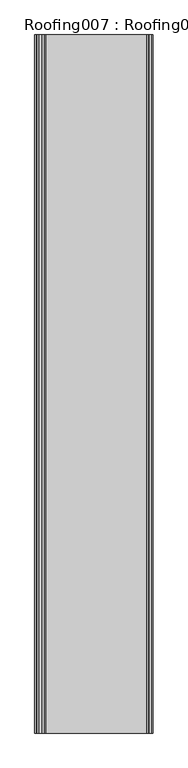
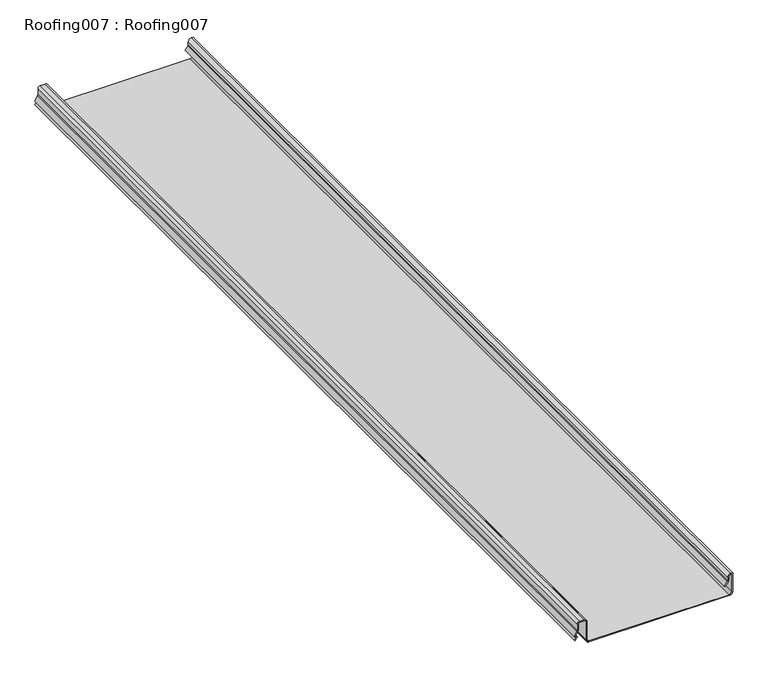
"""IFC4 building model written with IfcOpenShell, lengths in millimetres: proxy geometry, Roofing007 : Roofing007."""

from ifc_helpers import new_model, si_unit, point, frame, frame_2d, origin, place, context, project, spatial, polyline, circle_curve, trimmed, segment, composite_curve, outline, extrude, source, transform, mapped, element, save


def roofing007_roofing007_e383adbc(model_context):
    return source(origin(), model_context, "Body", "SweptSolid", [
        extrude(outline(composite_curve([segment(trimmed(circle_curve(frame_2d((42571.8416239, -858.0818689)), 5.08), [point((42568.8585944, -853.969943))], [point((42571.8416239, -853.0018689))], False, "CARTESIAN"), True, "CONTINUOUS"), segment(polyline([(42571.8416239, -853.0018689), (42578.5981823, -853.0018689)]), True, "CONTINUOUS"), segment(trimmed(circle_curve(frame_2d((42578.5981823, -847.9218689)), 5.08), [point((42578.5981823, -853.0018689))], [point((42583.6781823, -847.9218689))], True, "CARTESIAN"), True, "CONTINUOUS"), segment(polyline([(42583.6781823, -847.9218689), (42583.6781823, -846.3270642), (42543.9409948, -846.3270642)]), True, "CONTINUOUS"), segment(trimmed(circle_curve(frame_2d((42543.9409948, -851.4070642)), 5.08), [point((42543.9409948, -846.3270642))], [point((42538.8609948, -851.4070642))], True, "CARTESIAN"), True, "CONTINUOUS"), segment(polyline([(42538.8609948, -851.4070642), (42538.8609948, -1151.6811463)]), True, "CONTINUOUS"), segment(trimmed(circle_curve(frame_2d((42543.9409948, -1151.6811463)), 5.08), [point((42538.8609948, -1151.6811463))], [point((42543.9409948, -1156.7611463))], True, "CARTESIAN"), True, "CONTINUOUS"), segment(polyline([(42543.9409948, -1156.7611463), (42585.5544323, -1156.7611463)]), True, "CONTINUOUS"), segment(trimmed(circle_curve(frame_2d((42585.5544323, -1161.8411463)), 5.08), [point((42585.5544323, -1156.7611463))], [point((42590.6344323, -1161.8411463))], False, "CARTESIAN"), True, "CONTINUOUS"), segment(polyline([(42590.6344323, -1161.8411463), (42590.6344323, -1171.8489232)]), True, "CONTINUOUS"), segment(trimmed(circle_curve(frame_2d((42585.5544323, -1171.8489232)), 5.08), [point((42590.6344323, -1171.8489232))], [point((42585.5544323, -1176.9289232))], False, "CARTESIAN"), True, "CONTINUOUS"), segment(polyline([(42585.5544323, -1176.9289232), (42572.3718581, -1176.9289232)]), True, "CONTINUOUS"), segment(trimmed(circle_curve(frame_2d((42572.3718581, -1182.0089232)), 5.08), [point((42572.3718581, -1176.9289232))], [point((42569.8678467, -1177.5889315))], True, "CARTESIAN"), True, "CONTINUOUS"), segment(polyline([(42569.8678467, -1177.5889315), (42559.3102135, -1183.5700364), (42556.8688073, -1179.4059739), (42551.2672448, -1183.4049974), (42550.1051711, -1181.7772429), (42557.4874863, -1176.5069185), (42560.0388845, -1180.8585833), (42568.8820154, -1175.8487773)]), True, "CONTINUOUS"), segment(trimmed(circle_curve(frame_2d((42572.3718581, -1182.0089232)), 7.08), [point((42568.8820154, -1175.8487773))], [point((42572.3718581, -1174.9289232))], False, "CARTESIAN"), True, "CONTINUOUS"), segment(polyline([(42572.3718581, -1174.9289232), (42585.5544323, -1174.9289232)]), True, "CONTINUOUS"), segment(trimmed(circle_curve(frame_2d((42585.5544323, -1171.8489232)), 3.08), [point((42585.5544323, -1174.9289232))], [point((42588.6344323, -1171.8489232))], True, "CARTESIAN"), True, "CONTINUOUS"), segment(polyline([(42588.6344323, -1171.8489232), (42588.6344323, -1161.8411463)]), True, "CONTINUOUS"), segment(trimmed(circle_curve(frame_2d((42585.5544323, -1161.8411463)), 3.08), [point((42588.6344323, -1161.8411463))], [point((42585.5544323, -1158.7611463))], True, "CARTESIAN"), True, "CONTINUOUS"), segment(polyline([(42585.5544323, -1158.7611463), (42543.9409948, -1158.7611463)]), True, "CONTINUOUS"), segment(trimmed(circle_curve(frame_2d((42543.9409948, -1151.6811463)), 7.08), [point((42543.9409948, -1158.7611463))], [point((42536.8609948, -1151.6811463))], False, "CARTESIAN"), True, "CONTINUOUS"), segment(polyline([(42536.8609948, -1151.6811463), (42536.8609948, -851.4070642)]), True, "CONTINUOUS"), segment(trimmed(circle_curve(frame_2d((42543.9409948, -851.4070642)), 7.08), [point((42536.8609948, -851.4070642))], [point((42543.9409948, -844.3270642))], False, "CARTESIAN"), True, "CONTINUOUS"), segment(polyline([(42543.9409948, -844.3270642), (42585.6781823, -844.3270642), (42585.6781823, -847.9218689)]), True, "CONTINUOUS"), segment(trimmed(circle_curve(frame_2d((42578.5981823, -847.9218689)), 7.08), [point((42585.6781823, -847.9218689))], [point((42578.5981823, -855.0018689))], False, "CARTESIAN"), True, "CONTINUOUS"), segment(polyline([(42578.5981823, -855.0018689), (42571.8416239, -855.0018689)]), True, "CONTINUOUS"), segment(trimmed(circle_curve(frame_2d((42571.8416239, -858.0818689)), 3.08), [point((42571.8416239, -855.0018689))], [point((42570.0330155, -855.5888115))], True, "CARTESIAN"), True, "CONTINUOUS"), segment(polyline([(42570.0330155, -855.5888115), (42561.5588533, -861.7364601), (42560.3844323, -860.1175916), (42568.8585944, -853.969943)]), True, "CONTINUOUS")], self_intersect=False)), frame((0.0, -1052.8906574, 0.0), z_axis=(0.0, 1.0, 0.0), x_axis=(0.0, 0.0, 1.0)), (0.0, 0.0, 1.0), 2000.0),
    ])


if __name__ == "__main__":
    model = new_model("IFC4")
    model_context = context("Model", 3, world=origin())
    ifc_project = project(units=[si_unit("LENGTHUNIT", "METRE", prefix="MILLI")], contexts=[model_context])
    site = spatial("IfcSite", under=ifc_project)
    building = spatial("IfcBuilding", under=site)
    placement = place(None, origin())
    roofing007_roofing007_shape = roofing007_roofing007_e383adbc(model_context)
    element("IfcBuildingElementProxy", 1, Name="Roofing007 : Roofing007", ObjectType="Roofing007 : Roofing007", at=placement, inside=building, context=model_context, shape_type="MappedRepresentation", body=[
        mapped(roofing007_roofing007_shape, transform((0.0, 0.0, 0.0), x_axis=(1.0, 0.0, 0.0), y_axis=(0.0, 1.0, 0.0), z_axis=(0.0, 0.0, 1.0))),
    ])
    save(model, "model.ifc")

# Revit data of these elements
# Type "Roofing007 : Roofing007"
#   NameOverride = "Roofing007"
# Element 1 (IfcBuildingElementProxy, "Roofing007 : Roofing007")
#   Materials on its faces: "STANDING SEAM METAL ROOF"
# Materials
#   "STANDING SEAM METAL ROOF": class "Unassigned", colour RGB 128 128 128, transparency 0
